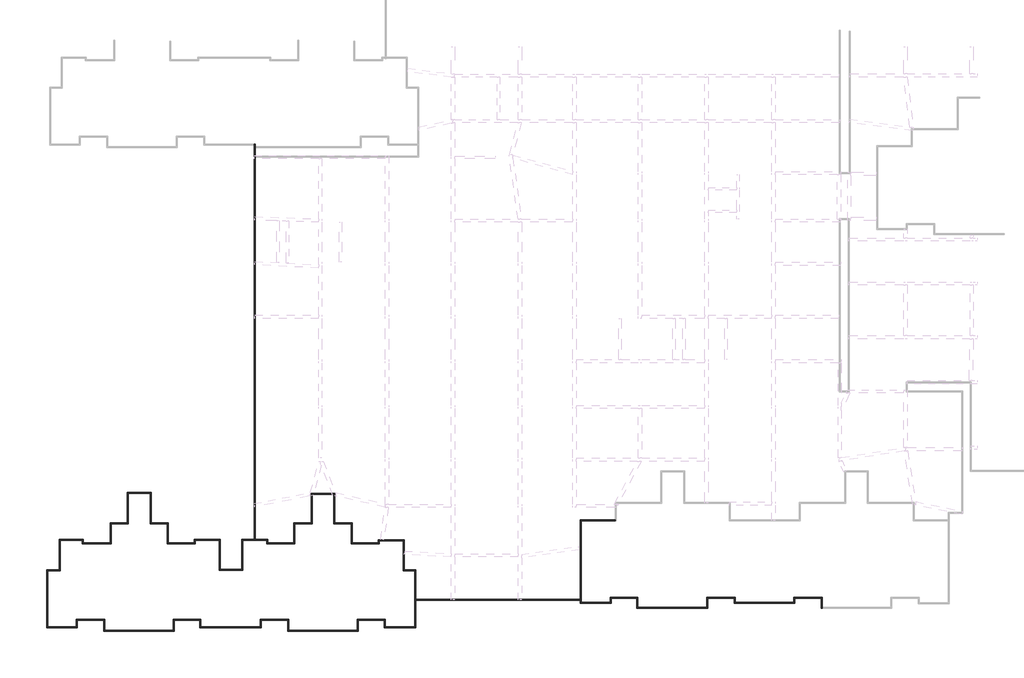
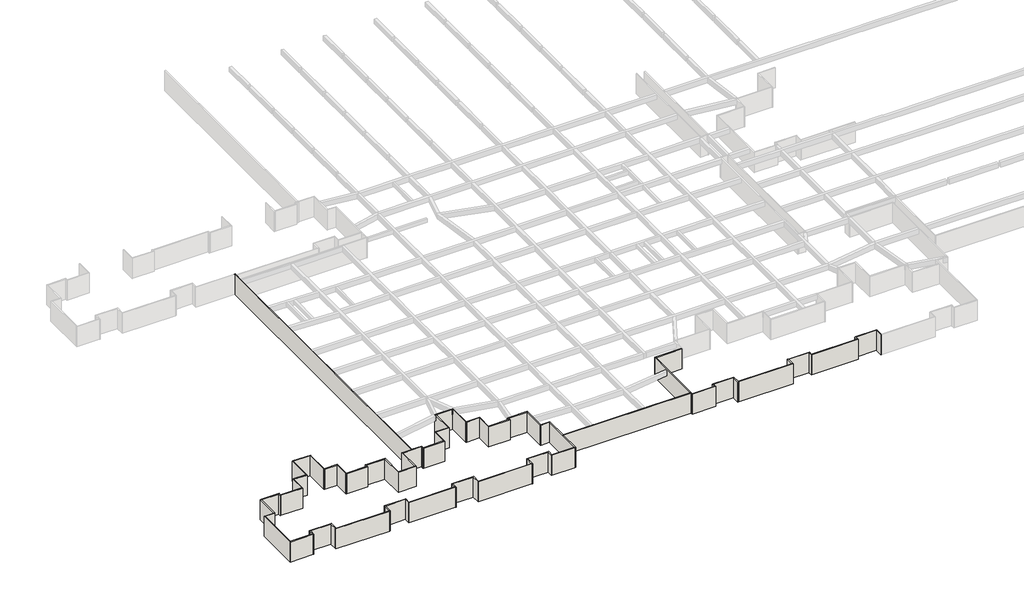
# One storey, part 1 of 16: 68 walls.
"""IFC4 building model written with IfcOpenShell, lengths in millimetres."""

from ifc_helpers import new_model, si_unit, origin, origin_with_axes, place, context, project, spatial, polyline, outline, extrude, faceted_brep, element, save

model = new_model("IFC4")

# Units and contexts
model_context = context("Model", 3, world=origin())
ifc_project = project(units=[si_unit("LENGTHUNIT", "METRE", prefix="MILLI")], contexts=[model_context])

# Site, building, storey
site = spatial("IfcSite", under=ifc_project)
building = spatial("IfcBuilding", under=site)
storey = spatial("IfcBuildingStorey", under=building, Name="户型图", Elevation=0.0)

# Walls
placement = place(None, origin())
element("IfcWall", 1, ObjectType="所有墙体", at=placement, inside=storey, context=model_context, shape_type="Brep", body=[
    faceted_brep([(223706.9772993, -230776.4067791, 0.0), (227415.8823447, -230776.4067791, 0.0), (227415.8823447, -230776.4067791, 3300.0), (223706.9772993, -230776.4067791, 3300.0), (223706.9772993, -230656.4067791, 0.0), (223706.9772993, -230656.4067791, 3300.0), (223826.9772993, -230656.4067791, 3300.0), (227295.8823447, -230656.4067791, 3300.0), (227415.8823447, -230656.4067791, 3300.0), (227415.8823447, -230656.4067791, 0.0), (227295.8823447, -230656.4067791, 0.0), (223826.9772993, -230656.4067791, 0.0)], [[[0, 1, 2, 3]], [[4, 5, 6, 7, 8, 9, 10, 11]], [[1, 0, 4, 11, 10, 9]], [[3, 2, 8, 7, 6, 5]], [[2, 1, 9, 8]], [[0, 3, 5, 4]]]),
])
element("IfcWall", 2, ObjectType="所有墙体", at=placement, inside=storey, context=model_context, shape_type="Brep", body=[
    faceted_brep([(227415.8823447, -230656.4067791, 0.0), (227415.8823447, -230192.9670343, 0.0), (227415.8823447, -230072.9670343, 0.0), (227415.8823447, -230072.9670343, 3300.0), (227415.8823447, -230192.9670343, 3300.0), (227415.8823447, -230656.4067791, 3300.0), (227295.8823447, -230656.4067791, 0.0), (227295.8823447, -230656.4067791, 3300.0), (227295.8823447, -230072.9670343, 3300.0), (227295.8823447, -230072.9670343, 0.0)], [[[0, 1, 2, 3, 4, 5]], [[6, 7, 8, 9]], [[2, 1, 0, 6, 9]], [[5, 4, 3, 8, 7]], [[0, 5, 7, 6]], [[3, 2, 9, 8]]]),
])
element("IfcWall", 3, ObjectType="所有墙体", at=placement, inside=storey, context=model_context, shape_type="Brep", body=[
    faceted_brep([(227415.8823447, -230192.9670343, 0.0), (230497.4582485, -230192.9670343, 0.0), (230617.4582485, -230192.9670343, 0.0), (230617.4582485, -230192.9670343, 3300.0), (230497.4582485, -230192.9670343, 3300.0), (227415.8823447, -230192.9670343, 3300.0), (227415.8823447, -230072.9670343, 0.0), (227415.8823447, -230072.9670343, 3300.0), (230617.4582485, -230072.9670343, 3300.0), (230617.4582485, -230072.9670343, 0.0)], [[[0, 1, 2, 3, 4, 5]], [[6, 7, 8, 9]], [[2, 1, 0, 6, 9]], [[5, 4, 3, 8, 7]], [[0, 5, 7, 6]], [[3, 2, 9, 8]]]),
])
element("IfcWall", 4, ObjectType="所有墙体", at=placement, inside=storey, context=model_context, shape_type="Brep", body=[
    faceted_brep([(230497.4582485, -230192.9670343, 0.0), (230497.4582485, -231395.926057, 0.0), (230497.4582485, -231395.926057, 3300.0), (230497.4582485, -230192.9670343, 3300.0), (230617.4582485, -230192.9670343, 0.0), (230617.4582485, -230192.9670343, 3300.0), (230617.4582485, -231275.926057, 3300.0), (230617.4582485, -231395.926057, 3300.0), (230617.4582485, -231395.926057, 0.0), (230617.4582485, -231275.926057, 0.0)], [[[0, 1, 2, 3]], [[4, 5, 6, 7, 8, 9]], [[1, 0, 4, 9, 8]], [[3, 2, 7, 6, 5]], [[0, 3, 5, 4]], [[2, 1, 8, 7]]]),
])
element("IfcWall", 5, ObjectType="所有墙体", at=placement, inside=storey, context=model_context, shape_type="Brep", body=[
    faceted_brep([(230617.4582485, -231395.926057, 0.0), (239114.4178107, -231395.926057, 0.0), (239114.4178107, -231395.926057, 3300.0), (230617.4582485, -231395.926057, 3300.0), (230617.4582485, -231275.926057, 0.0), (230617.4582485, -231275.926057, 3300.0), (238994.4178107, -231275.926057, 3300.0), (239114.4178107, -231275.926057, 3300.0), (239114.4178107, -231275.926057, 0.0), (238994.4178107, -231275.926057, 0.0)], [[[0, 1, 2, 3]], [[4, 5, 6, 7, 8, 9]], [[1, 0, 4, 9, 8]], [[3, 2, 7, 6, 5]], [[0, 3, 5, 4]], [[2, 1, 8, 7]]]),
])
element("IfcWall", 6, ObjectType="所有墙体", at=placement, inside=storey, context=model_context, shape_type="Brep", body=[
    faceted_brep([(239114.4178107, -231275.926057, 0.0), (239114.4178107, -230192.9670343, 0.0), (239114.4178107, -230072.9670343, 0.0), (239114.4178107, -230072.9670343, 3300.0), (239114.4178107, -230192.9670343, 3300.0), (239114.4178107, -231275.926057, 3300.0), (238994.4178107, -231275.926057, 0.0), (238994.4178107, -231275.926057, 3300.0), (238994.4178107, -230072.9670343, 3300.0), (238994.4178107, -230072.9670343, 0.0)], [[[0, 1, 2, 3, 4, 5]], [[6, 7, 8, 9]], [[2, 1, 0, 6, 9]], [[5, 4, 3, 8, 7]], [[0, 5, 7, 6]], [[3, 2, 9, 8]]]),
])
element("IfcWall", 7, ObjectType="所有墙体", at=placement, inside=storey, context=model_context, shape_type="Brep", body=[
    faceted_brep([(239114.4178107, -230192.9670343, 0.0), (242297.4654708, -230192.9670343, 0.0), (242417.4654708, -230192.9670343, 0.0), (242417.4654708, -230192.9670343, 3300.0), (242297.4654708, -230192.9670343, 3300.0), (239114.4178107, -230192.9670343, 3300.0), (239114.4178107, -230072.9670343, 0.0), (239114.4178107, -230072.9670343, 3300.0), (242417.4654708, -230072.9670343, 3300.0), (242417.4654708, -230072.9670343, 0.0)], [[[0, 1, 2, 3, 4, 5]], [[6, 7, 8, 9]], [[2, 1, 0, 6, 9]], [[5, 4, 3, 8, 7]], [[0, 5, 7, 6]], [[3, 2, 9, 8]]]),
])
element("IfcWall", 8, ObjectType="所有墙体", at=placement, inside=storey, context=model_context, shape_type="Brep", body=[
    faceted_brep([(242297.4654708, -230192.9670343, 0.0), (242297.4654708, -230776.4067791, 0.0), (242297.4654708, -230776.4067791, 3300.0), (242297.4654708, -230192.9670343, 3300.0), (242417.4654708, -230192.9670343, 0.0), (242417.4654708, -230192.9670343, 3300.0), (242417.4654708, -230656.4067791, 3300.0), (242417.4654708, -230776.4067791, 3300.0), (242417.4654708, -230776.4067791, 0.0), (242417.4654708, -230656.4067791, 0.0)], [[[0, 1, 2, 3]], [[4, 5, 6, 7, 8, 9]], [[1, 0, 4, 9, 8]], [[3, 2, 7, 6, 5]], [[0, 3, 5, 4]], [[2, 1, 8, 7]]]),
])
element("IfcWall", 9, ObjectType="所有墙体", at=placement, inside=storey, context=model_context, shape_type="Brep", body=[
    faceted_brep([(242417.4654708, -230776.4067791, 0.0), (249616.6616196, -230776.4067791, 0.0), (249616.6616196, -230776.4067791, 3300.0), (242417.4654708, -230776.4067791, 3300.0), (242417.4654708, -230656.4067791, 0.0), (242417.4654708, -230656.4067791, 3300.0), (249496.6616196, -230656.4067791, 3300.0), (249616.6616196, -230656.4067791, 3300.0), (249616.6616196, -230656.4067791, 0.0), (249496.6616196, -230656.4067791, 0.0)], [[[0, 1, 2, 3]], [[4, 5, 6, 7, 8, 9]], [[1, 0, 4, 9, 8]], [[3, 2, 7, 6, 5]], [[0, 3, 5, 4]], [[2, 1, 8, 7]]]),
])
element("IfcWall", 10, ObjectType="所有墙体", at=placement, inside=storey, context=model_context, shape_type="Brep", body=[
    faceted_brep([(249616.6616196, -230656.4067791, 0.0), (249616.6616196, -230192.9670343, 0.0), (249616.6616196, -230072.9670343, 0.0), (249616.6616196, -230072.9670343, 3300.0), (249616.6616196, -230192.9670343, 3300.0), (249616.6616196, -230656.4067791, 3300.0), (249496.6616196, -230656.4067791, 0.0), (249496.6616196, -230656.4067791, 3300.0), (249496.6616196, -230072.9670343, 3300.0), (249496.6616196, -230072.9670343, 0.0)], [[[0, 1, 2, 3, 4, 5]], [[6, 7, 8, 9]], [[2, 1, 0, 6, 9]], [[5, 4, 3, 8, 7]], [[0, 5, 7, 6]], [[3, 2, 9, 8]]]),
])
element("IfcWall", 11, ObjectType="所有墙体", at=placement, inside=storey, context=model_context, shape_type="Brep", body=[
    faceted_brep([(249616.6616196, -230192.9670343, 0.0), (252797.4720082, -230192.9670343, 0.0), (252917.4720082, -230192.9670343, 0.0), (252917.4720082, -230192.9670343, 3300.0), (252797.4720082, -230192.9670343, 3300.0), (249616.6616196, -230192.9670343, 3300.0), (249616.6616196, -230072.9670343, 0.0), (249616.6616196, -230072.9670343, 3300.0), (252917.4720082, -230072.9670343, 3300.0), (252917.4720082, -230072.9670343, 0.0)], [[[0, 1, 2, 3, 4, 5]], [[6, 7, 8, 9]], [[2, 1, 0, 6, 9]], [[5, 4, 3, 8, 7]], [[0, 5, 7, 6]], [[3, 2, 9, 8]]]),
])
element("IfcWall", 12, ObjectType="所有墙体", at=placement, inside=storey, context=model_context, shape_type="Brep", body=[
    faceted_brep([(252797.4720082, -230192.9670343, 0.0), (252797.4720082, -231395.926057, 0.0), (252797.4720082, -231395.926057, 3300.0), (252797.4720082, -230192.9670343, 3300.0), (252917.4720082, -230192.9670343, 0.0), (252917.4720082, -230192.9670343, 3300.0), (252917.4720082, -231275.926057, 3300.0), (252917.4720082, -231395.926057, 3300.0), (252917.4720082, -231395.926057, 0.0), (252917.4720082, -231275.926057, 0.0)], [[[0, 1, 2, 3]], [[4, 5, 6, 7, 8, 9]], [[1, 0, 4, 9, 8]], [[3, 2, 7, 6, 5]], [[0, 3, 5, 4]], [[2, 1, 8, 7]]]),
])
element("IfcWall", 13, ObjectType="所有墙体", at=placement, inside=storey, context=model_context, shape_type="Brep", body=[
    faceted_brep([(227909.4754658, -220713.7545432, 0.0), (223706.9772993, -220713.7545432, 0.0), (223706.9772993, -220713.7545432, 3300.0), (227909.4754658, -220713.7545432, 3300.0), (227909.4754658, -220833.7545432, 0.0), (227909.4754658, -220833.7545432, 3300.0), (223826.9772993, -220833.7545432, 3300.0), (223706.9772993, -220833.7545432, 3300.0), (223706.9772993, -220833.7545432, 0.0), (223826.9772993, -220833.7545432, 0.0)], [[[0, 1, 2, 3]], [[4, 5, 6, 7, 8, 9]], [[1, 0, 4, 9, 8]], [[3, 2, 7, 6, 5]], [[0, 3, 5, 4]], [[2, 1, 8, 7]]]),
])
element("IfcWall", 14, ObjectType="所有墙体", at=placement, inside=storey, context=model_context, shape_type="Brep", body=[
    faceted_brep([(223706.9772993, -220833.7545432, 0.0), (223706.9772993, -230332.9670343, 0.0), (223706.9772993, -230452.9670343, 0.0), (223706.9772993, -230656.4067791, 0.0), (223706.9772993, -230656.4067791, 3300.0), (223706.9772993, -230452.9670343, 3300.0), (223706.9772993, -230332.9670343, 3300.0), (223706.9772993, -220833.7545432, 3300.0), (223826.9772993, -220833.7545432, 0.0), (223826.9772993, -220833.7545432, 3300.0), (223826.9772993, -230656.4067791, 3300.0), (223826.9772993, -230656.4067791, 0.0)], [[[0, 1, 2, 3, 4, 5, 6, 7]], [[8, 9, 10, 11]], [[3, 2, 1, 0, 8, 11]], [[7, 6, 5, 4, 10, 9]], [[4, 3, 11, 10]], [[0, 7, 9, 8]]]),
])
element("IfcWall", 15, ObjectType="所有墙体", at=placement, inside=storey, context=model_context, shape_type="SweptSolid", body=[
    extrude(outline(polyline([(203826.9772993, -230332.9670343), (223706.9772993, -230332.9670343), (223706.9772993, -230452.9670343), (203826.9772993, -230452.9670343), (203826.9772993, -230332.9670343)])), origin_with_axes(), (0.0, 0.0, 1.0), 3300.0),
])
element("IfcWall", 16, ObjectType="所有墙体", at=placement, inside=storey, context=model_context, shape_type="Brep", body=[
    faceted_brep([(203706.9772993, -226864.0850951, 0.0), (203706.9772993, -233644.4703624, 0.0), (203706.9772993, -233764.4703624, 0.0), (203706.9772993, -233764.4703624, 3300.0), (203706.9772993, -233644.4703624, 3300.0), (203706.9772993, -226864.0850951, 3300.0), (203826.9772993, -226864.0850951, 0.0), (203826.9772993, -226864.0850951, 3300.0), (203826.9772993, -230332.9670343, 3300.0), (203826.9772993, -230452.9670343, 3300.0), (203826.9772993, -233764.4703624, 3300.0), (203826.9772993, -233764.4703624, 0.0), (203826.9772993, -230452.9670343, 0.0), (203826.9772993, -230332.9670343, 0.0)], [[[0, 1, 2, 3, 4, 5]], [[6, 7, 8, 9, 10, 11, 12, 13]], [[2, 1, 0, 6, 13, 12, 11]], [[5, 4, 3, 10, 9, 8, 7]], [[3, 2, 11, 10]], [[0, 5, 7, 6]]]),
])
element("IfcWall", 17, ObjectType="所有墙体", at=placement, inside=storey, context=model_context, shape_type="Brep", body=[
    faceted_brep([(203706.9772993, -233644.4703624, 0.0), (200175.3999887, -233644.4703624, 0.0), (200055.3999887, -233644.4703624, 0.0), (200055.3999887, -233644.4703624, 3300.0), (200175.3999887, -233644.4703624, 3300.0), (203706.9772993, -233644.4703624, 3300.0), (203706.9772993, -233764.4703624, 0.0), (203706.9772993, -233764.4703624, 3300.0), (200055.3999887, -233764.4703624, 3300.0), (200055.3999887, -233764.4703624, 0.0)], [[[0, 1, 2, 3, 4, 5]], [[6, 7, 8, 9]], [[2, 1, 0, 6, 9]], [[5, 4, 3, 8, 7]], [[0, 5, 7, 6]], [[3, 2, 9, 8]]]),
])
element("IfcWall", 18, ObjectType="所有墙体", at=placement, inside=storey, context=model_context, shape_type="Brep", body=[
    faceted_brep([(200175.3999887, -233644.4703624, 0.0), (200175.3999887, -232740.7855886, 0.0), (200175.3999887, -232740.7855886, 3300.0), (200175.3999887, -233644.4703624, 3300.0), (200055.3999887, -233644.4703624, 0.0), (200055.3999887, -233644.4703624, 3300.0), (200055.3999887, -232860.7855886, 3300.0), (200055.3999887, -232740.7855886, 3300.0), (200055.3999887, -232740.7855886, 0.0), (200055.3999887, -232860.7855886, 0.0)], [[[0, 1, 2, 3]], [[4, 5, 6, 7, 8, 9]], [[1, 0, 4, 9, 8]], [[3, 2, 7, 6, 5]], [[0, 3, 5, 4]], [[2, 1, 8, 7]]]),
])
element("IfcWall", 19, ObjectType="所有墙体", at=placement, inside=storey, context=model_context, shape_type="Brep", body=[
    faceted_brep([(200055.3999887, -232740.7855886, 0.0), (196755.597577, -232740.7855886, 0.0), (196755.597577, -232740.7855886, 3300.0), (200055.3999887, -232740.7855886, 3300.0), (200055.3999887, -232860.7855886, 0.0), (200055.3999887, -232860.7855886, 3300.0), (196875.597577, -232860.7855886, 3300.0), (196755.597577, -232860.7855886, 3300.0), (196755.597577, -232860.7855886, 0.0), (196875.597577, -232860.7855886, 0.0)], [[[0, 1, 2, 3]], [[4, 5, 6, 7, 8, 9]], [[1, 0, 4, 9, 8]], [[3, 2, 7, 6, 5]], [[0, 3, 5, 4]], [[2, 1, 8, 7]]]),
])
element("IfcWall", 20, ObjectType="所有墙体", at=placement, inside=storey, context=model_context, shape_type="Brep", body=[
    faceted_brep([(196755.597577, -232860.7855886, 0.0), (196755.597577, -234037.6063178, 0.0), (196755.597577, -234157.6063178, 0.0), (196755.597577, -234157.6063178, 3300.0), (196755.597577, -234037.6063178, 3300.0), (196755.597577, -232860.7855886, 3300.0), (196875.597577, -232860.7855886, 0.0), (196875.597577, -232860.7855886, 3300.0), (196875.597577, -234157.6063178, 3300.0), (196875.597577, -234157.6063178, 0.0)], [[[0, 1, 2, 3, 4, 5]], [[6, 7, 8, 9]], [[2, 1, 0, 6, 9]], [[5, 4, 3, 8, 7]], [[0, 5, 7, 6]], [[3, 2, 9, 8]]]),
])
element("IfcWall", 21, ObjectType="所有墙体", at=placement, inside=storey, context=model_context, shape_type="Brep", body=[
    faceted_brep([(196755.597577, -234037.6063178, 0.0), (188474.9819031, -234037.6063178, 0.0), (188354.9819031, -234037.6063178, 0.0), (188354.9819031, -234037.6063178, 3300.0), (188474.9819031, -234037.6063178, 3300.0), (196755.597577, -234037.6063178, 3300.0), (196755.597577, -234157.6063178, 0.0), (196755.597577, -234157.6063178, 3300.0), (188354.9819031, -234157.6063178, 3300.0), (188354.9819031, -234157.6063178, 0.0)], [[[0, 1, 2, 3, 4, 5]], [[6, 7, 8, 9]], [[2, 1, 0, 6, 9]], [[5, 4, 3, 8, 7]], [[0, 5, 7, 6]], [[3, 2, 9, 8]]]),
])
element("IfcWall", 22, ObjectType="所有墙体", at=placement, inside=storey, context=model_context, shape_type="Brep", body=[
    faceted_brep([(188474.9819031, -234037.6063178, 0.0), (188474.9819031, -232740.7855886, 0.0), (188474.9819031, -232740.7855886, 3300.0), (188474.9819031, -234037.6063178, 3300.0), (188354.9819031, -234037.6063178, 0.0), (188354.9819031, -234037.6063178, 3300.0), (188354.9819031, -232860.7855886, 3300.0), (188354.9819031, -232740.7855886, 3300.0), (188354.9819031, -232740.7855886, 0.0), (188354.9819031, -232860.7855886, 0.0)], [[[0, 1, 2, 3]], [[4, 5, 6, 7, 8, 9]], [[1, 0, 4, 9, 8]], [[3, 2, 7, 6, 5]], [[0, 3, 5, 4]], [[2, 1, 8, 7]]]),
])
element("IfcWall", 23, ObjectType="所有墙体", at=placement, inside=storey, context=model_context, shape_type="Brep", body=[
    faceted_brep([(188354.9819031, -232740.7855886, 0.0), (185055.2276269, -232740.7855886, 0.0), (185055.2276269, -232740.7855886, 3300.0), (188354.9819031, -232740.7855886, 3300.0), (188354.9819031, -232860.7855886, 0.0), (188354.9819031, -232860.7855886, 3300.0), (185175.2276269, -232860.7855886, 3300.0), (185055.2276269, -232860.7855886, 3300.0), (185055.2276269, -232860.7855886, 0.0), (185175.2276269, -232860.7855886, 0.0)], [[[0, 1, 2, 3]], [[4, 5, 6, 7, 8, 9]], [[1, 0, 4, 9, 8]], [[3, 2, 7, 6, 5]], [[0, 3, 5, 4]], [[2, 1, 8, 7]]]),
])
element("IfcWall", 24, ObjectType="所有墙体", at=placement, inside=storey, context=model_context, shape_type="Brep", body=[
    faceted_brep([(185055.2276269, -232860.7855886, 0.0), (185055.2276269, -233644.4703624, 0.0), (185055.2276269, -233764.4703624, 0.0), (185055.2276269, -233764.4703624, 3300.0), (185055.2276269, -233644.4703624, 3300.0), (185055.2276269, -232860.7855886, 3300.0), (185175.2276269, -232860.7855886, 0.0), (185175.2276269, -232860.7855886, 3300.0), (185175.2276269, -233764.4703624, 3300.0), (185175.2276269, -233764.4703624, 0.0)], [[[0, 1, 2, 3, 4, 5]], [[6, 7, 8, 9]], [[2, 1, 0, 6, 9]], [[5, 4, 3, 8, 7]], [[0, 5, 7, 6]], [[3, 2, 9, 8]]]),
])
element("IfcWall", 25, ObjectType="所有墙体", at=placement, inside=storey, context=model_context, shape_type="Brep", body=[
    faceted_brep([(185055.2276269, -233644.4703624, 0.0), (177874.9677687, -233644.4703624, 0.0), (177754.9677687, -233644.4703624, 0.0), (177754.9677687, -233644.4703624, 3300.0), (177874.9677687, -233644.4703624, 3300.0), (185055.2276269, -233644.4703624, 3300.0), (185055.2276269, -233764.4703624, 0.0), (185055.2276269, -233764.4703624, 3300.0), (177754.9677687, -233764.4703624, 3300.0), (177754.9677687, -233764.4703624, 0.0)], [[[0, 1, 2, 3, 4, 5]], [[6, 7, 8, 9]], [[2, 1, 0, 6, 9]], [[5, 4, 3, 8, 7]], [[0, 5, 7, 6]], [[3, 2, 9, 8]]]),
])
element("IfcWall", 26, ObjectType="所有墙体", at=placement, inside=storey, context=model_context, shape_type="Brep", body=[
    faceted_brep([(177874.9677687, -233644.4703624, 0.0), (177874.9677687, -232740.7855886, 0.0), (177874.9677687, -232740.7855886, 3300.0), (177874.9677687, -233644.4703624, 3300.0), (177754.9677687, -233644.4703624, 0.0), (177754.9677687, -233644.4703624, 3300.0), (177754.9677687, -232860.7855886, 3300.0), (177754.9677687, -232740.7855886, 3300.0), (177754.9677687, -232740.7855886, 0.0), (177754.9677687, -232860.7855886, 0.0)], [[[0, 1, 2, 3]], [[4, 5, 6, 7, 8, 9]], [[1, 0, 4, 9, 8]], [[3, 2, 7, 6, 5]], [[0, 3, 5, 4]], [[2, 1, 8, 7]]]),
])
element("IfcWall", 27, ObjectType="所有墙体", at=placement, inside=storey, context=model_context, shape_type="Brep", body=[
    faceted_brep([(177754.9677687, -232740.7855886, 0.0), (174555.583755, -232740.7855886, 0.0), (174555.583755, -232740.7855886, 3300.0), (177754.9677687, -232740.7855886, 3300.0), (177754.9677687, -232860.7855886, 0.0), (177754.9677687, -232860.7855886, 3300.0), (174675.583755, -232860.7855886, 3300.0), (174555.583755, -232860.7855886, 3300.0), (174555.583755, -232860.7855886, 0.0), (174675.583755, -232860.7855886, 0.0)], [[[0, 1, 2, 3]], [[4, 5, 6, 7, 8, 9]], [[1, 0, 4, 9, 8]], [[3, 2, 7, 6, 5]], [[0, 3, 5, 4]], [[2, 1, 8, 7]]]),
])
element("IfcWall", 28, ObjectType="所有墙体", at=placement, inside=storey, context=model_context, shape_type="Brep", body=[
    faceted_brep([(174555.583755, -232860.7855886, 0.0), (174555.583755, -234037.6063178, 0.0), (174555.583755, -234157.6063178, 0.0), (174555.583755, -234157.6063178, 3300.0), (174555.583755, -234037.6063178, 3300.0), (174555.583755, -232860.7855886, 3300.0), (174675.583755, -232860.7855886, 0.0), (174675.583755, -232860.7855886, 3300.0), (174675.583755, -234157.6063178, 3300.0), (174675.583755, -234157.6063178, 0.0)], [[[0, 1, 2, 3, 4, 5]], [[6, 7, 8, 9]], [[2, 1, 0, 6, 9]], [[5, 4, 3, 8, 7]], [[0, 5, 7, 6]], [[3, 2, 9, 8]]]),
])
element("IfcWall", 29, ObjectType="所有墙体", at=placement, inside=storey, context=model_context, shape_type="Brep", body=[
    faceted_brep([(174555.583755, -234037.6063178, 0.0), (166275.583755, -234037.6063178, 0.0), (166155.583755, -234037.6063178, 0.0), (166155.583755, -234037.6063178, 3300.0), (166275.583755, -234037.6063178, 3300.0), (174555.583755, -234037.6063178, 3300.0), (174555.583755, -234157.6063178, 0.0), (174555.583755, -234157.6063178, 3300.0), (166155.583755, -234157.6063178, 3300.0), (166155.583755, -234157.6063178, 0.0)], [[[0, 1, 2, 3, 4, 5]], [[6, 7, 8, 9]], [[2, 1, 0, 6, 9]], [[5, 4, 3, 8, 7]], [[0, 5, 7, 6]], [[3, 2, 9, 8]]]),
])
element("IfcWall", 30, ObjectType="所有墙体", at=placement, inside=storey, context=model_context, shape_type="Brep", body=[
    faceted_brep([(166275.583755, -234037.6063178, 0.0), (166275.583755, -232740.7855886, 0.0), (166275.583755, -232740.7855886, 3300.0), (166275.583755, -234037.6063178, 3300.0), (166155.583755, -234037.6063178, 0.0), (166155.583755, -234037.6063178, 3300.0), (166155.583755, -232860.7855886, 3300.0), (166155.583755, -232740.7855886, 3300.0), (166155.583755, -232740.7855886, 0.0), (166155.583755, -232860.7855886, 0.0)], [[[0, 1, 2, 3]], [[4, 5, 6, 7, 8, 9]], [[1, 0, 4, 9, 8]], [[3, 2, 7, 6, 5]], [[0, 3, 5, 4]], [[2, 1, 8, 7]]]),
])
element("IfcWall", 31, ObjectType="所有墙体", at=placement, inside=storey, context=model_context, shape_type="Brep", body=[
    faceted_brep([(166155.583755, -232740.7855886, 0.0), (162855.771752, -232740.7855886, 0.0), (162855.771752, -232740.7855886, 3300.0), (166155.583755, -232740.7855886, 3300.0), (166155.583755, -232860.7855886, 0.0), (166155.583755, -232860.7855886, 3300.0), (162975.771752, -232860.7855886, 3300.0), (162855.771752, -232860.7855886, 3300.0), (162855.771752, -232860.7855886, 0.0), (162975.771752, -232860.7855886, 0.0)], [[[0, 1, 2, 3]], [[4, 5, 6, 7, 8, 9]], [[1, 0, 4, 9, 8]], [[3, 2, 7, 6, 5]], [[0, 3, 5, 4]], [[2, 1, 8, 7]]]),
])
element("IfcWall", 32, ObjectType="所有墙体", at=placement, inside=storey, context=model_context, shape_type="Brep", body=[
    faceted_brep([(162855.771752, -232860.7855886, 0.0), (162855.771752, -233644.4703624, 0.0), (162855.771752, -233764.4703624, 0.0), (162855.771752, -233764.4703624, 3300.0), (162855.771752, -233644.4703624, 3300.0), (162855.771752, -232860.7855886, 3300.0), (162975.771752, -232860.7855886, 0.0), (162975.771752, -232860.7855886, 3300.0), (162975.771752, -233764.4703624, 3300.0), (162975.771752, -233764.4703624, 0.0)], [[[0, 1, 2, 3, 4, 5]], [[6, 7, 8, 9]], [[2, 1, 0, 6, 9]], [[5, 4, 3, 8, 7]], [[0, 5, 7, 6]], [[3, 2, 9, 8]]]),
])
element("IfcWall", 33, ObjectType="所有墙体", at=placement, inside=storey, context=model_context, shape_type="Brep", body=[
    faceted_brep([(162855.771752, -233644.4703624, 0.0), (159373.4496687, -233644.4703624, 0.0), (159253.4496687, -233644.4703624, 0.0), (159253.4496687, -233644.4703624, 3300.0), (159373.4496687, -233644.4703624, 3300.0), (162855.771752, -233644.4703624, 3300.0), (162855.771752, -233764.4703624, 0.0), (162855.771752, -233764.4703624, 3300.0), (159253.4496687, -233764.4703624, 3300.0), (159253.4496687, -233764.4703624, 0.0)], [[[0, 1, 2, 3, 4, 5]], [[6, 7, 8, 9]], [[2, 1, 0, 6, 9]], [[5, 4, 3, 8, 7]], [[0, 5, 7, 6]], [[3, 2, 9, 8]]]),
])
element("IfcWall", 34, ObjectType="所有墙体", at=placement, inside=storey, context=model_context, shape_type="Brep", body=[
    faceted_brep([(159373.4496687, -233644.4703624, 0.0), (159373.4496687, -226864.4703624, 0.0), (159373.4496687, -226744.4703624, 0.0), (159373.4496687, -226744.4703624, 3300.0), (159373.4496687, -226864.4703624, 3300.0), (159373.4496687, -233644.4703624, 3300.0), (159253.4496687, -233644.4703624, 0.0), (159253.4496687, -233644.4703624, 3300.0), (159253.4496687, -226744.4703624, 3300.0), (159253.4496687, -226744.4703624, 0.0)], [[[0, 1, 2, 3, 4, 5]], [[6, 7, 8, 9]], [[2, 1, 0, 6, 9]], [[5, 4, 3, 8, 7]], [[0, 5, 7, 6]], [[3, 2, 9, 8]]]),
])
element("IfcWall", 35, ObjectType="所有墙体", at=placement, inside=storey, context=model_context, shape_type="Brep", body=[
    faceted_brep([(159373.4496687, -226864.4703624, 0.0), (160883.9958696, -226864.4703624, 0.0), (160883.9958696, -226864.4703624, 3300.0), (159373.4496687, -226864.4703624, 3300.0), (159373.4496687, -226744.4703624, 0.0), (159373.4496687, -226744.4703624, 3300.0), (160763.9958696, -226744.4703624, 3300.0), (160883.9958696, -226744.4703624, 3300.0), (160883.9958696, -226744.4703624, 0.0), (160763.9958696, -226744.4703624, 0.0)], [[[0, 1, 2, 3]], [[4, 5, 6, 7, 8, 9]], [[1, 0, 4, 9, 8]], [[3, 2, 7, 6, 5]], [[0, 3, 5, 4]], [[2, 1, 8, 7]]]),
])
element("IfcWall", 36, ObjectType="所有墙体", at=placement, inside=storey, context=model_context, shape_type="Brep", body=[
    faceted_brep([(160883.9958696, -226744.4703624, 0.0), (160883.9958696, -223216.850594, 0.0), (160883.9958696, -223096.850594, 0.0), (160883.9958696, -223096.850594, 3300.0), (160883.9958696, -223216.850594, 3300.0), (160883.9958696, -226744.4703624, 3300.0), (160763.9958696, -226744.4703624, 0.0), (160763.9958696, -226744.4703624, 3300.0), (160763.9958696, -223096.850594, 3300.0), (160763.9958696, -223096.850594, 0.0)], [[[0, 1, 2, 3, 4, 5]], [[6, 7, 8, 9]], [[2, 1, 0, 6, 9]], [[5, 4, 3, 8, 7]], [[0, 5, 7, 6]], [[3, 2, 9, 8]]]),
])
element("IfcWall", 37, ObjectType="所有墙体", at=placement, inside=storey, context=model_context, shape_type="Brep", body=[
    faceted_brep([(160883.9958696, -223216.850594, 0.0), (163563.9958696, -223216.850594, 0.0), (163683.9958696, -223216.850594, 0.0), (163683.9958696, -223216.850594, 3300.0), (163563.9958696, -223216.850594, 3300.0), (160883.9958696, -223216.850594, 3300.0), (160883.9958696, -223096.850594, 0.0), (160883.9958696, -223096.850594, 3300.0), (163683.9958696, -223096.850594, 3300.0), (163683.9958696, -223096.850594, 0.0)], [[[0, 1, 2, 3, 4, 5]], [[6, 7, 8, 9]], [[2, 1, 0, 6, 9]], [[5, 4, 3, 8, 7]], [[0, 5, 7, 6]], [[3, 2, 9, 8]]]),
])
element("IfcWall", 38, ObjectType="所有墙体", at=placement, inside=storey, context=model_context, shape_type="Brep", body=[
    faceted_brep([(163563.9958696, -223216.850594, 0.0), (163563.9958696, -223622.1234451, 0.0), (163563.9958696, -223622.1234451, 3300.0), (163563.9958696, -223216.850594, 3300.0), (163683.9958696, -223216.850594, 0.0), (163683.9958696, -223216.850594, 3300.0), (163683.9958696, -223502.1234451, 3300.0), (163683.9958696, -223622.1234451, 3300.0), (163683.9958696, -223622.1234451, 0.0), (163683.9958696, -223502.1234451, 0.0)], [[[0, 1, 2, 3]], [[4, 5, 6, 7, 8, 9]], [[1, 0, 4, 9, 8]], [[3, 2, 7, 6, 5]], [[0, 3, 5, 4]], [[2, 1, 8, 7]]]),
])
element("IfcWall", 39, ObjectType="所有墙体", at=placement, inside=storey, context=model_context, shape_type="Brep", body=[
    faceted_brep([(163683.9958696, -223622.1234451, 0.0), (167083.9958696, -223622.1234451, 0.0), (167083.9958696, -223622.1234451, 3300.0), (163683.9958696, -223622.1234451, 3300.0), (163683.9958696, -223502.1234451, 0.0), (163683.9958696, -223502.1234451, 3300.0), (166963.9958696, -223502.1234451, 3300.0), (167083.9958696, -223502.1234451, 3300.0), (167083.9958696, -223502.1234451, 0.0), (166963.9958696, -223502.1234451, 0.0)], [[[0, 1, 2, 3]], [[4, 5, 6, 7, 8, 9]], [[1, 0, 4, 9, 8]], [[3, 2, 7, 6, 5]], [[0, 3, 5, 4]], [[2, 1, 8, 7]]]),
])
element("IfcWall", 40, ObjectType="所有墙体", at=placement, inside=storey, context=model_context, shape_type="Brep", body=[
    faceted_brep([(167083.9958696, -223502.1234451, 0.0), (167083.9958696, -221223.7957944, 0.0), (167083.9958696, -221103.7957944, 0.0), (167083.9958696, -221103.7957944, 3300.0), (167083.9958696, -221223.7957944, 3300.0), (167083.9958696, -223502.1234451, 3300.0), (166963.9958696, -223502.1234451, 0.0), (166963.9958696, -223502.1234451, 3300.0), (166963.9958696, -221103.7957944, 3300.0), (166963.9958696, -221103.7957944, 0.0)], [[[0, 1, 2, 3, 4, 5]], [[6, 7, 8, 9]], [[2, 1, 0, 6, 9]], [[5, 4, 3, 8, 7]], [[0, 5, 7, 6]], [[3, 2, 9, 8]]]),
])
element("IfcWall", 41, ObjectType="所有墙体", at=placement, inside=storey, context=model_context, shape_type="Brep", body=[
    faceted_brep([(167083.9958696, -221223.7957944, 0.0), (169140.5185226, -221223.7957944, 0.0), (169140.5185226, -221223.7957944, 3300.0), (167083.9958696, -221223.7957944, 3300.0), (167083.9958696, -221103.7957944, 0.0), (167083.9958696, -221103.7957944, 3300.0), (169020.5185226, -221103.7957944, 3300.0), (169140.5185226, -221103.7957944, 3300.0), (169140.5185226, -221103.7957944, 0.0), (169020.5185226, -221103.7957944, 0.0)], [[[0, 1, 2, 3]], [[4, 5, 6, 7, 8, 9]], [[1, 0, 4, 9, 8]], [[3, 2, 7, 6, 5]], [[0, 3, 5, 4]], [[2, 1, 8, 7]]]),
])
element("IfcWall", 42, ObjectType="所有墙体", at=placement, inside=storey, context=model_context, shape_type="Brep", body=[
    faceted_brep([(169140.5185226, -221103.7957944, 0.0), (169140.5185226, -217528.1551832, 0.0), (169140.5185226, -217408.1551832, 0.0), (169140.5185226, -217408.1551832, 3300.0), (169140.5185226, -217528.1551832, 3300.0), (169140.5185226, -221103.7957944, 3300.0), (169020.5185226, -221103.7957944, 0.0), (169020.5185226, -221103.7957944, 3300.0), (169020.5185226, -217408.1551832, 3300.0), (169020.5185226, -217408.1551832, 0.0)], [[[0, 1, 2, 3, 4, 5]], [[6, 7, 8, 9]], [[2, 1, 0, 6, 9]], [[5, 4, 3, 8, 7]], [[0, 5, 7, 6]], [[3, 2, 9, 8]]]),
])
element("IfcWall", 43, ObjectType="所有墙体", at=placement, inside=storey, context=model_context, shape_type="Brep", body=[
    faceted_brep([(169140.5185226, -217528.1551832, 0.0), (171768.3939286, -217528.1551832, 0.0), (171888.3939286, -217528.1551832, 0.0), (171888.3939286, -217528.1551832, 3300.0), (171768.3939286, -217528.1551832, 3300.0), (169140.5185226, -217528.1551832, 3300.0), (169140.5185226, -217408.1551832, 0.0), (169140.5185226, -217408.1551832, 3300.0), (171888.3939286, -217408.1551832, 3300.0), (171888.3939286, -217408.1551832, 0.0)], [[[0, 1, 2, 3, 4, 5]], [[6, 7, 8, 9]], [[2, 1, 0, 6, 9]], [[5, 4, 3, 8, 7]], [[0, 5, 7, 6]], [[3, 2, 9, 8]]]),
])
element("IfcWall", 44, ObjectType="所有墙体", at=placement, inside=storey, context=model_context, shape_type="Brep", body=[
    faceted_brep([(171768.3939286, -217528.1551832, 0.0), (171768.3939286, -221223.7957944, 0.0), (171768.3939286, -221223.7957944, 3300.0), (171768.3939286, -217528.1551832, 3300.0), (171888.3939286, -217528.1551832, 0.0), (171888.3939286, -217528.1551832, 3300.0), (171888.3939286, -221103.7957944, 3300.0), (171888.3939286, -221223.7957944, 3300.0), (171888.3939286, -221223.7957944, 0.0), (171888.3939286, -221103.7957944, 0.0)], [[[0, 1, 2, 3]], [[4, 5, 6, 7, 8, 9]], [[1, 0, 4, 9, 8]], [[3, 2, 7, 6, 5]], [[0, 3, 5, 4]], [[2, 1, 8, 7]]]),
])
element("IfcWall", 45, ObjectType="所有墙体", at=placement, inside=storey, context=model_context, shape_type="Brep", body=[
    faceted_brep([(171888.3939286, -221223.7957944, 0.0), (173817.5367432, -221223.7957944, 0.0), (173937.5367432, -221223.7957944, 0.0), (173937.5367432, -221223.7957944, 3300.0), (173817.5367432, -221223.7957944, 3300.0), (171888.3939286, -221223.7957944, 3300.0), (171888.3939286, -221103.7957944, 0.0), (171888.3939286, -221103.7957944, 3300.0), (173937.5367432, -221103.7957944, 3300.0), (173937.5367432, -221103.7957944, 0.0)], [[[0, 1, 2, 3, 4, 5]], [[6, 7, 8, 9]], [[2, 1, 0, 6, 9]], [[5, 4, 3, 8, 7]], [[0, 5, 7, 6]], [[3, 2, 9, 8]]]),
])
element("IfcWall", 46, ObjectType="所有墙体", at=placement, inside=storey, context=model_context, shape_type="Brep", body=[
    faceted_brep([(173817.5367432, -221223.7957944, 0.0), (173817.5367432, -223622.1234451, 0.0), (173817.5367432, -223622.1234451, 3300.0), (173817.5367432, -221223.7957944, 3300.0), (173937.5367432, -221223.7957944, 0.0), (173937.5367432, -221223.7957944, 3300.0), (173937.5367432, -223502.1234451, 3300.0), (173937.5367432, -223622.1234451, 3300.0), (173937.5367432, -223622.1234451, 0.0), (173937.5367432, -223502.1234451, 0.0)], [[[0, 1, 2, 3]], [[4, 5, 6, 7, 8, 9]], [[1, 0, 4, 9, 8]], [[3, 2, 7, 6, 5]], [[0, 3, 5, 4]], [[2, 1, 8, 7]]]),
])
element("IfcWall", 47, ObjectType="所有墙体", at=placement, inside=storey, context=model_context, shape_type="Brep", body=[
    faceted_brep([(173937.5367432, -223622.1234451, 0.0), (177235.7830045, -223622.1234451, 0.0), (177235.7830045, -223622.1234451, 3300.0), (173937.5367432, -223622.1234451, 3300.0), (173937.5367432, -223502.1234451, 0.0), (173937.5367432, -223502.1234451, 3300.0), (177115.7830045, -223502.1234451, 3300.0), (177235.7830045, -223502.1234451, 3300.0), (177235.7830045, -223502.1234451, 0.0), (177115.7830045, -223502.1234451, 0.0)], [[[0, 1, 2, 3]], [[4, 5, 6, 7, 8, 9]], [[1, 0, 4, 9, 8]], [[3, 2, 7, 6, 5]], [[0, 3, 5, 4]], [[2, 1, 8, 7]]]),
])
element("IfcWall", 48, ObjectType="所有墙体", at=placement, inside=storey, context=model_context, shape_type="Brep", body=[
    faceted_brep([(177235.7830045, -223502.1234451, 0.0), (177235.7830045, -223216.850594, 0.0), (177235.7830045, -223096.850594, 0.0), (177235.7830045, -223096.850594, 3300.0), (177235.7830045, -223216.850594, 3300.0), (177235.7830045, -223502.1234451, 3300.0), (177115.7830045, -223502.1234451, 0.0), (177115.7830045, -223502.1234451, 3300.0), (177115.7830045, -223096.850594, 3300.0), (177115.7830045, -223096.850594, 0.0)], [[[0, 1, 2, 3, 4, 5]], [[6, 7, 8, 9]], [[2, 1, 0, 6, 9]], [[5, 4, 3, 8, 7]], [[0, 5, 7, 6]], [[3, 2, 9, 8]]]),
])
element("IfcWall", 49, ObjectType="所有墙体", at=placement, inside=storey, context=model_context, shape_type="Brep", body=[
    faceted_brep([(177235.7830045, -223216.850594, 0.0), (180116.2371142, -223216.850594, 0.0), (180236.2371142, -223216.850594, 0.0), (180236.2371142, -223216.850594, 3300.0), (180116.2371142, -223216.850594, 3300.0), (177235.7830045, -223216.850594, 3300.0), (177235.7830045, -223096.850594, 0.0), (177235.7830045, -223096.850594, 3300.0), (180236.2371142, -223096.850594, 3300.0), (180236.2371142, -223096.850594, 0.0)], [[[0, 1, 2, 3, 4, 5]], [[6, 7, 8, 9]], [[2, 1, 0, 6, 9]], [[5, 4, 3, 8, 7]], [[0, 5, 7, 6]], [[3, 2, 9, 8]]]),
])
element("IfcWall", 50, ObjectType="所有墙体", at=placement, inside=storey, context=model_context, shape_type="Brep", body=[
    faceted_brep([(180116.2371142, -223216.850594, 0.0), (180116.2371142, -226838.699103, 0.0), (180116.2371142, -226838.699103, 3300.0), (180116.2371142, -223216.850594, 3300.0), (180236.2371142, -223216.850594, 0.0), (180236.2371142, -223216.850594, 3300.0), (180236.2371142, -226718.699103, 3300.0), (180236.2371142, -226838.699103, 3300.0), (180236.2371142, -226838.699103, 0.0), (180236.2371142, -226718.699103, 0.0)], [[[0, 1, 2, 3]], [[4, 5, 6, 7, 8, 9]], [[1, 0, 4, 9, 8]], [[3, 2, 7, 6, 5]], [[0, 3, 5, 4]], [[2, 1, 8, 7]]]),
])
element("IfcWall", 51, ObjectType="所有墙体", at=placement, inside=storey, context=model_context, shape_type="Brep", body=[
    faceted_brep([(180236.2371142, -226838.699103, 0.0), (182932.1971931, -226838.699103, 0.0), (182932.1971931, -226838.699103, 3300.0), (180236.2371142, -226838.699103, 3300.0), (180236.2371142, -226718.699103, 0.0), (180236.2371142, -226718.699103, 3300.0), (182812.1971931, -226718.699103, 3300.0), (182932.1971931, -226718.699103, 3300.0), (182932.1971931, -226718.699103, 0.0), (182812.1971931, -226718.699103, 0.0)], [[[0, 1, 2, 3]], [[4, 5, 6, 7, 8, 9]], [[1, 0, 4, 9, 8]], [[3, 2, 7, 6, 5]], [[0, 3, 5, 4]], [[2, 1, 8, 7]]]),
])
element("IfcWall", 52, ObjectType="所有墙体", at=placement, inside=storey, context=model_context, shape_type="Brep", body=[
    faceted_brep([(182932.1971931, -226718.699103, 0.0), (182932.1971931, -223216.850594, 0.0), (182932.1971931, -223096.850594, 0.0), (182932.1971931, -223096.850594, 3300.0), (182932.1971931, -223216.850594, 3300.0), (182932.1971931, -226718.699103, 3300.0), (182812.1971931, -226718.699103, 0.0), (182812.1971931, -226718.699103, 3300.0), (182812.1971931, -223096.850594, 3300.0), (182812.1971931, -223096.850594, 0.0)], [[[0, 1, 2, 3, 4, 5]], [[6, 7, 8, 9]], [[2, 1, 0, 6, 9]], [[5, 4, 3, 8, 7]], [[0, 5, 7, 6]], [[3, 2, 9, 8]]]),
])
element("IfcWall", 53, ObjectType="所有墙体", at=placement, inside=storey, context=model_context, shape_type="Brep", body=[
    faceted_brep([(182932.1971931, -223216.850594, 0.0), (185816.2406631, -223216.850594, 0.0), (185936.2406631, -223216.850594, 0.0), (185936.2406631, -223216.850594, 3300.0), (185816.2406631, -223216.850594, 3300.0), (182932.1971931, -223216.850594, 3300.0), (182932.1971931, -223096.850594, 0.0), (182932.1971931, -223096.850594, 3300.0), (184314.2189281, -223096.850594, 3300.0), (184434.2189281, -223096.850594, 3300.0), (185936.2406631, -223096.850594, 3300.0), (185936.2406631, -223096.850594, 0.0), (184434.2189281, -223096.850594, 0.0), (184314.2189281, -223096.850594, 0.0)], [[[0, 1, 2, 3, 4, 5]], [[6, 7, 8, 9, 10, 11, 12, 13]], [[2, 1, 0, 6, 13, 12, 11]], [[5, 4, 3, 10, 9, 8, 7]], [[0, 5, 7, 6]], [[3, 2, 11, 10]]]),
])
element("IfcWall", 54, ObjectType="所有墙体", at=placement, inside=storey, context=model_context, shape_type="Brep", body=[
    faceted_brep([(185816.2406631, -223216.850594, 0.0), (185816.2406631, -223622.1234451, 0.0), (185816.2406631, -223622.1234451, 3300.0), (185816.2406631, -223216.850594, 3300.0), (185936.2406631, -223216.850594, 0.0), (185936.2406631, -223216.850594, 3300.0), (185936.2406631, -223502.1234451, 3300.0), (185936.2406631, -223622.1234451, 3300.0), (185936.2406631, -223622.1234451, 0.0), (185936.2406631, -223502.1234451, 0.0)], [[[0, 1, 2, 3]], [[4, 5, 6, 7, 8, 9]], [[1, 0, 4, 9, 8]], [[3, 2, 7, 6, 5]], [[0, 3, 5, 4]], [[2, 1, 8, 7]]]),
])
element("IfcWall", 55, ObjectType="所有墙体", at=placement, inside=storey, context=model_context, shape_type="Brep", body=[
    faceted_brep([(185936.2406631, -223622.1234451, 0.0), (189235.7607746, -223622.1234451, 0.0), (189235.7607746, -223622.1234451, 3300.0), (185936.2406631, -223622.1234451, 3300.0), (185936.2406631, -223502.1234451, 0.0), (185936.2406631, -223502.1234451, 3300.0), (189115.7607746, -223502.1234451, 3300.0), (189235.7607746, -223502.1234451, 3300.0), (189235.7607746, -223502.1234451, 0.0), (189115.7607746, -223502.1234451, 0.0)], [[[0, 1, 2, 3]], [[4, 5, 6, 7, 8, 9]], [[1, 0, 4, 9, 8]], [[3, 2, 7, 6, 5]], [[0, 3, 5, 4]], [[2, 1, 8, 7]]]),
])
element("IfcWall", 56, ObjectType="所有墙体", at=placement, inside=storey, context=model_context, shape_type="Brep", body=[
    faceted_brep([(189235.7607746, -223502.1234451, 0.0), (189235.7607746, -221223.7957944, 0.0), (189235.7607746, -221103.7957944, 0.0), (189235.7607746, -221103.7957944, 3300.0), (189235.7607746, -221223.7957944, 3300.0), (189235.7607746, -223502.1234451, 3300.0), (189115.7607746, -223502.1234451, 0.0), (189115.7607746, -223502.1234451, 3300.0), (189115.7607746, -221103.7957944, 3300.0), (189115.7607746, -221103.7957944, 0.0)], [[[0, 1, 2, 3, 4, 5]], [[6, 7, 8, 9]], [[2, 1, 0, 6, 9]], [[5, 4, 3, 8, 7]], [[0, 5, 7, 6]], [[3, 2, 9, 8]]]),
])
element("IfcWall", 57, ObjectType="所有墙体", at=placement, inside=storey, context=model_context, shape_type="Brep", body=[
    faceted_brep([(189235.7607746, -221223.7957944, 0.0), (191338.4680648, -221223.7957944, 0.0), (191338.4680648, -221223.7957944, 3300.0), (189235.7607746, -221223.7957944, 3300.0), (189235.7607746, -221103.7957944, 0.0), (189235.7607746, -221103.7957944, 3300.0), (191218.4680648, -221103.7957944, 3300.0), (191338.4680648, -221103.7957944, 3300.0), (191338.4680648, -221103.7957944, 0.0), (191218.4680648, -221103.7957944, 0.0)], [[[0, 1, 2, 3]], [[4, 5, 6, 7, 8, 9]], [[1, 0, 4, 9, 8]], [[3, 2, 7, 6, 5]], [[0, 3, 5, 4]], [[2, 1, 8, 7]]]),
])
element("IfcWall", 58, ObjectType="所有墙体", at=placement, inside=storey, context=model_context, shape_type="Brep", body=[
    faceted_brep([(191338.4680648, -221103.7957944, 0.0), (191338.4680648, -217650.8034485, 0.0), (191338.4680648, -217530.8034485, 0.0), (191338.4680648, -217530.8034485, 3300.0), (191338.4680648, -217650.8034485, 3300.0), (191338.4680648, -221103.7957944, 3300.0), (191218.4680648, -221103.7957944, 0.0), (191218.4680648, -221103.7957944, 3300.0), (191218.4680648, -217530.8034485, 3300.0), (191218.4680648, -217530.8034485, 0.0)], [[[0, 1, 2, 3, 4, 5]], [[6, 7, 8, 9]], [[2, 1, 0, 6, 9]], [[5, 4, 3, 8, 7]], [[0, 5, 7, 6]], [[3, 2, 9, 8]]]),
])
element("IfcWall", 59, ObjectType="所有墙体", at=placement, inside=storey, context=model_context, shape_type="Brep", body=[
    faceted_brep([(191338.4680648, -217650.8034485, 0.0), (193922.0585089, -217650.8034485, 0.0), (194042.0585089, -217650.8034485, 0.0), (194042.0585089, -217650.8034485, 3300.0), (193922.0585089, -217650.8034485, 3300.0), (191338.4680648, -217650.8034485, 3300.0), (191338.4680648, -217530.8034485, 0.0), (191338.4680648, -217530.8034485, 3300.0), (194042.0585089, -217530.8034485, 3300.0), (194042.0585089, -217530.8034485, 0.0)], [[[0, 1, 2, 3, 4, 5]], [[6, 7, 8, 9]], [[2, 1, 0, 6, 9]], [[5, 4, 3, 8, 7]], [[0, 5, 7, 6]], [[3, 2, 9, 8]]]),
])
element("IfcWall", 60, ObjectType="所有墙体", at=placement, inside=storey, context=model_context, shape_type="Brep", body=[
    faceted_brep([(193922.0585089, -217650.8034485, 0.0), (193922.0585089, -221223.7957944, 0.0), (193922.0585089, -221223.7957944, 3300.0), (193922.0585089, -217650.8034485, 3300.0), (194042.0585089, -217650.8034485, 0.0), (194042.0585089, -217650.8034485, 3300.0), (194042.0585089, -221103.7957944, 3300.0), (194042.0585089, -221223.7957944, 3300.0), (194042.0585089, -221223.7957944, 0.0), (194042.0585089, -221103.7957944, 0.0)], [[[0, 1, 2, 3]], [[4, 5, 6, 7, 8, 9]], [[1, 0, 4, 9, 8]], [[3, 2, 7, 6, 5]], [[0, 3, 5, 4]], [[2, 1, 8, 7]]]),
])
element("IfcWall", 61, ObjectType="所有墙体", at=placement, inside=storey, context=model_context, shape_type="Brep", body=[
    faceted_brep([(194042.0585089, -221223.7957944, 0.0), (196018.4710534, -221223.7957944, 0.0), (196138.4710534, -221223.7957944, 0.0), (196138.4710534, -221223.7957944, 3300.0), (196018.4710534, -221223.7957944, 3300.0), (194042.0585089, -221223.7957944, 3300.0), (194042.0585089, -221103.7957944, 0.0), (194042.0585089, -221103.7957944, 3300.0), (196138.4710534, -221103.7957944, 3300.0), (196138.4710534, -221103.7957944, 0.0)], [[[0, 1, 2, 3, 4, 5]], [[6, 7, 8, 9]], [[2, 1, 0, 6, 9]], [[5, 4, 3, 8, 7]], [[0, 5, 7, 6]], [[3, 2, 9, 8]]]),
])
element("IfcWall", 62, ObjectType="所有墙体", at=placement, inside=storey, context=model_context, shape_type="Brep", body=[
    faceted_brep([(196018.4710534, -221223.7957944, 0.0), (196018.4710534, -223622.1234451, 0.0), (196018.4710534, -223622.1234451, 3300.0), (196018.4710534, -221223.7957944, 3300.0), (196138.4710534, -221223.7957944, 0.0), (196138.4710534, -221223.7957944, 3300.0), (196138.4710534, -223502.1234451, 3300.0), (196138.4710534, -223622.1234451, 3300.0), (196138.4710534, -223622.1234451, 0.0), (196138.4710534, -223502.1234451, 0.0)], [[[0, 1, 2, 3]], [[4, 5, 6, 7, 8, 9]], [[1, 0, 4, 9, 8]], [[3, 2, 7, 6, 5]], [[0, 3, 5, 4]], [[2, 1, 8, 7]]]),
])
element("IfcWall", 63, ObjectType="所有墙体", at=placement, inside=storey, context=model_context, shape_type="Brep", body=[
    faceted_brep([(196138.4710534, -223622.1234451, 0.0), (199435.7968264, -223622.1234451, 0.0), (199435.7968264, -223622.1234451, 3300.0), (196138.4710534, -223622.1234451, 3300.0), (196138.4710534, -223502.1234451, 0.0), (196138.4710534, -223502.1234451, 3300.0), (199315.7968264, -223502.1234451, 3300.0), (199435.7968264, -223502.1234451, 3300.0), (199435.7968264, -223502.1234451, 0.0), (199315.7968264, -223502.1234451, 0.0)], [[[0, 1, 2, 3]], [[4, 5, 6, 7, 8, 9]], [[1, 0, 4, 9, 8]], [[3, 2, 7, 6, 5]], [[0, 3, 5, 4]], [[2, 1, 8, 7]]]),
])
element("IfcWall", 64, ObjectType="所有墙体", at=placement, inside=storey, context=model_context, shape_type="Brep", body=[
    faceted_brep([(199435.7968264, -223502.1234451, 0.0), (199435.7968264, -223259.2388283, 0.0), (199435.7968264, -223139.2388283, 0.0), (199435.7968264, -223139.2388283, 3300.0), (199435.7968264, -223259.2388283, 3300.0), (199435.7968264, -223502.1234451, 3300.0), (199315.7968264, -223502.1234451, 0.0), (199315.7968264, -223502.1234451, 3300.0), (199315.7968264, -223139.2388283, 3300.0), (199315.7968264, -223139.2388283, 0.0)], [[[0, 1, 2, 3, 4, 5]], [[6, 7, 8, 9]], [[2, 1, 0, 6, 9]], [[5, 4, 3, 8, 7]], [[0, 5, 7, 6]], [[3, 2, 9, 8]]]),
])
element("IfcWall", 65, ObjectType="所有墙体", at=placement, inside=storey, context=model_context, shape_type="Brep", body=[
    faceted_brep([(199435.7968264, -223259.2388283, 0.0), (202315.7968264, -223259.2388283, 0.0), (202435.7968264, -223259.2388283, 0.0), (202435.7968264, -223259.2388283, 3300.0), (202315.7968264, -223259.2388283, 3300.0), (199435.7968264, -223259.2388283, 3300.0), (199435.7968264, -223139.2388283, 0.0), (199435.7968264, -223139.2388283, 3300.0), (202435.7968264, -223139.2388283, 3300.0), (202435.7968264, -223139.2388283, 0.0)], [[[0, 1, 2, 3, 4, 5]], [[6, 7, 8, 9]], [[2, 1, 0, 6, 9]], [[5, 4, 3, 8, 7]], [[0, 5, 7, 6]], [[3, 2, 9, 8]]]),
])
element("IfcWall", 66, ObjectType="所有墙体", at=placement, inside=storey, context=model_context, shape_type="Brep", body=[
    faceted_brep([(202315.7968264, -223259.2388283, 0.0), (202315.7968264, -226864.0850951, 0.0), (202315.7968264, -226864.0850951, 3300.0), (202315.7968264, -223259.2388283, 3300.0), (202435.7968264, -223259.2388283, 0.0), (202435.7968264, -223259.2388283, 3300.0), (202435.7968264, -226744.0850951, 3300.0), (202435.7968264, -226864.0850951, 3300.0), (202435.7968264, -226864.0850951, 0.0), (202435.7968264, -226744.0850951, 0.0)], [[[0, 1, 2, 3]], [[4, 5, 6, 7, 8, 9]], [[1, 0, 4, 9, 8]], [[3, 2, 7, 6, 5]], [[0, 3, 5, 4]], [[2, 1, 8, 7]]]),
])
element("IfcWall", 67, ObjectType="所有墙体", at=placement, inside=storey, context=model_context, shape_type="Brep", body=[
    faceted_brep([(202435.7968264, -226864.0850951, 0.0), (203706.9772993, -226864.0850951, 0.0), (203826.9772993, -226864.0850951, 0.0), (203826.9772993, -226864.0850951, 3300.0), (203706.9772993, -226864.0850951, 3300.0), (202435.7968264, -226864.0850951, 3300.0), (202435.7968264, -226744.0850951, 0.0), (202435.7968264, -226744.0850951, 3300.0), (203826.9772993, -226744.0850951, 3300.0), (203826.9772993, -226744.0850951, 0.0)], [[[0, 1, 2, 3, 4, 5]], [[6, 7, 8, 9]], [[2, 1, 0, 6, 9]], [[5, 4, 3, 8, 7]], [[0, 5, 7, 6]], [[3, 2, 9, 8]]]),
])
element("IfcWall", 68, ObjectType="所有墙体", at=placement, inside=storey, context=model_context, shape_type="Brep", body=[
    faceted_brep([(184434.2189281, -223096.850594, 0.0), (184434.2189281, -176865.1471774, 0.0), (184434.2189281, -176745.1471774, 0.0), (184434.2189281, -175750.7737405, 0.0), (184434.2189281, -175630.7737405, 0.0), (184434.2189281, -175296.850594, 0.0), (184434.2189281, -175296.850594, 3300.0), (184434.2189281, -175630.7737405, 3300.0), (184434.2189281, -175750.7737405, 3300.0), (184434.2189281, -176745.1471774, 3300.0), (184434.2189281, -176865.1471774, 3300.0), (184434.2189281, -223096.850594, 3300.0), (184314.2189281, -223096.850594, 0.0), (184314.2189281, -223096.850594, 3300.0), (184314.2189281, -175416.850594, 3300.0), (184314.2189281, -175296.850594, 3300.0), (184314.2189281, -175296.850594, 0.0), (184314.2189281, -175416.850594, 0.0)], [[[0, 1, 2, 3, 4, 5, 6, 7, 8, 9, 10, 11]], [[12, 13, 14, 15, 16, 17]], [[5, 4, 3, 2, 1, 0, 12, 17, 16]], [[11, 10, 9, 8, 7, 6, 15, 14, 13]], [[0, 11, 13, 12]], [[6, 5, 16, 15]]]),
])

save(model, "model.ifc")

# Revit data of these elements
# Project information
#   项目发布日期 = "出图日期"
#   项目状态 = "项目状态"
#   客户姓名 = "所有者"
#   项目地址 = "## 街道\n省市自治区邮政编码"
#   项目名称 = "项目名称"
#   项目编号 = "项目编号"
# Type "所有墙体"
#   Layers, outside or top first: 120 mm "默认" (function 1)
# Elements 1, 2, 3, 4, 5, 6, 7, 8, 9, 10, 11, 12, 13, 14, 15, 16, 17, 18, 19, 20, 21, 22, 23, 24, 25, 26, 27, 28, 29, 30, 31, 32, 33, 34, 35, 36, 37, 38, 39, 40, 41, 42, 43, 44, 45, 46, 47, 48, 49, 50, 51, 52, 53, 54, 55, 56, 57, 58, 59, 60, 61, 62, 63, 64, 65, 66, 67, 68 (IfcWall, "所有墙体")
#   Top Offset = 0 mm
#   Base Offset = 0 mm
#   wall height = 3300 mm
#   Phase Created = 新构造
#   Base Constraint = 户型图
#   Top Constraint = 层高
#   Materials on its faces: "默认"
# Materials
#   "默认": class "其他", colour RGB 192 192 192, transparency 0, Cost = 0
# Area at (183573.558, -170449.512) mm, upper offset 0 mm, lower offset 0 mm
#   Number = "170"
#   Name = "main_building"
# Area, not placed, upper offset 0 mm, lower offset 0 mm
#   Number = "80"
#   Name = "main_building"
# Area, not placed, upper offset 0 mm, lower offset 0 mm
#   Number = "118"
#   Name = "main_building"
# Area, not placed, upper offset 0 mm, lower offset 0 mm
#   Number = "160"
#   Name = "fire_compart"
# Area, not placed, upper offset 0 mm, lower offset 0 mm
#   Number = "149"
#   Name = "main_building"
# Area, not placed, upper offset 0 mm, lower offset 0 mm
#   Number = "81"
#   Name = "fire_compart"
# Area, not placed, upper offset 0 mm, lower offset 0 mm
#   Number = "82"
#   Name = "main_building"
# Area, not placed, upper offset 0 mm, lower offset 0 mm
#   Number = "91"
#   Name = "main_building"
# Area, not placed, upper offset 0 mm, lower offset 0 mm
#   Number = "31"
#   Name = "main_building"
# Area, not placed, upper offset 0 mm, lower offset 0 mm
#   Number = "32"
#   Name = "main_building"
# Area, not placed, upper offset 0 mm, lower offset 0 mm
#   Number = "33"
#   Name = "main_building"
# Area, not placed, upper offset 0 mm, lower offset 0 mm
#   Number = "34"
#   Name = "main_building"
# Area, not placed, upper offset 0 mm, lower offset 0 mm
#   Number = "35"
#   Name = "main_building"
# Area, not placed, upper offset 0 mm, lower offset 0 mm
#   Number = "41"
#   Name = "main_building"
# Area, not placed, upper offset 0 mm, lower offset 0 mm
#   Number = "42"
#   Name = "main_building"
# Area, not placed, upper offset 0 mm, lower offset 0 mm
#   Number = "43"
#   Name = "main_building"
# Area, not placed, upper offset 0 mm, lower offset 0 mm
#   Number = "44"
#   Name = "main_building"
# Area, not placed, upper offset 0 mm, lower offset 0 mm
#   Number = "45"
#   Name = "main_building"
# Area, not placed, upper offset 0 mm, lower offset 0 mm
#   Number = "46"
#   Name = "main_building"
# Area, not placed, upper offset 0 mm, lower offset 0 mm
#   Number = "47"
#   Name = "main_building"
# Area, not placed, upper offset 0 mm, lower offset 0 mm
#   Number = "48"
#   Name = "main_building"
# Area, not placed, upper offset 0 mm, lower offset 0 mm
#   Number = "49"
#   Name = "main_building"
# Area, not placed, upper offset 0 mm, lower offset 0 mm
#   Number = "50"
#   Name = "main_building"
# Area, not placed, upper offset 0 mm, lower offset 0 mm
#   Number = "5"
#   Name = "fire_compart_3"
# Area, not placed, upper offset 0 mm, lower offset 0 mm
#   Number = "119"
#   Name = "main_building"
# Area, not placed, upper offset 0 mm, lower offset 0 mm
#   Number = "9"
#   Name = "main_building"
# Area, not placed, upper offset 0 mm, lower offset 0 mm
#   Number = "10"
#   Name = "main_building"
# Area, not placed, upper offset 0 mm, lower offset 0 mm
#   Number = "11"
#   Name = "main_building"
# Area, not placed, upper offset 0 mm, lower offset 0 mm
#   Number = "51"
#   Name = "fire_compart"
# Area, not placed, upper offset 0 mm, lower offset 0 mm
#   Number = "12"
#   Name = "main_building"
# Area, not placed, upper offset 0 mm, lower offset 0 mm
#   Number = "157"
#   Name = "fire_compart"
# Area, not placed, upper offset 0 mm, lower offset 0 mm
#   Number = "158"
#   Name = "fire_compart"
# Area, not placed, upper offset 0 mm, lower offset 0 mm
#   Number = "13"
#   Name = "main_building"
# Area, not placed, upper offset 0 mm, lower offset 0 mm
#   Number = "14"
#   Name = "main_building"
# Area, not placed, upper offset 0 mm, lower offset 0 mm
#   Number = "15"
#   Name = "main_building"
# Area, not placed, upper offset 0 mm, lower offset 0 mm
#   Number = "16"
#   Name = "main_building"
# Area, not placed, upper offset 0 mm, lower offset 0 mm
#   Number = "17"
#   Name = "main_building"
# Area, not placed, upper offset 0 mm, lower offset 0 mm
#   Number = "18"
#   Name = "main_building"
# Area, not placed, upper offset 0 mm, lower offset 0 mm
#   Number = "19"
#   Name = "面积"
# Area, not placed, upper offset 0 mm, lower offset 0 mm
#   Number = "20"
#   Name = "main_building"
# Area, not placed, upper offset 0 mm, lower offset 0 mm
#   Number = "21"
#   Name = "main_building"
# Area, not placed, upper offset 0 mm, lower offset 0 mm
#   Number = "22"
#   Name = "main_building"
# Area, not placed, upper offset 0 mm, lower offset 0 mm
#   Number = "107"
#   Name = "main_building"
# Area, not placed, upper offset 0 mm, lower offset 0 mm
#   Number = "120"
#   Name = "main_building"
# Area, not placed, upper offset 0 mm, lower offset 0 mm
#   Number = "74"
#   Name = "main_building"
# Room, not placed, phase "新构造", upper offset 0 mm, lower offset 0 mm
#   Number = "9"
#   Name = "客餐厅轮廓"
# Area, not placed, upper offset 0 mm, lower offset 0 mm
#   Number = "92"
#   Name = "fire_compart"
# Area, not placed, upper offset 0 mm, lower offset 0 mm
#   Number = "93"
#   Name = "main_building"
# Area, not placed, upper offset 0 mm, lower offset 0 mm
#   Number = "94"
#   Name = "main_building"
# Room, not placed, phase "新构造", upper offset 0 mm, lower offset 0 mm
#   Number = "10"
#   Name = "墙面轮廓"
# Area at (453200.583, -173539.101) mm, upper offset 0 mm, lower offset 0 mm
#   Number = "165"
#   Name = "main_building"
# Area, not placed, upper offset 0 mm, lower offset 0 mm
#   Number = "52"
#   Name = "fire_compart"
# Area, not placed, upper offset 0 mm, lower offset 0 mm
#   Number = "53"
#   Name = "fire_compart"
# Area, not placed, upper offset 0 mm, lower offset 0 mm
#   Number = "102"
#   Name = "main_building"
# Area, not placed, upper offset 0 mm, lower offset 0 mm
#   Number = "121"
#   Name = "main_building"
# Area, not placed, upper offset 0 mm, lower offset 0 mm
#   Number = "54"
#   Name = "fire_compart"
# Area, not placed, upper offset 0 mm, lower offset 0 mm
#   Number = "95"
#   Name = "fire_compart"
# Area, not placed, upper offset 0 mm, lower offset 0 mm
#   Number = "96"
#   Name = "main_building"
# Area, not placed, upper offset 0 mm, lower offset 0 mm
#   Number = "97"
#   Name = "main_building"
# Area, not placed, upper offset 0 mm, lower offset 0 mm
#   Number = "122"
#   Name = "main_building"
# Area, not placed, upper offset 0 mm, lower offset 0 mm
#   Number = "148"
#   Name = "main_building"
# Area, not placed, upper offset 0 mm, lower offset 0 mm
#   Number = "6"
#   Name = "fire_compart_4"
# Area, not placed, upper offset 0 mm, lower offset 0 mm
#   Number = "55"
#   Name = "fire_compart"
# Area, not placed, upper offset 0 mm, lower offset 0 mm
#   Number = "56"
#   Name = "fire_compart"
# Area, not placed, upper offset 0 mm, lower offset 0 mm
#   Number = "142"
#   Name = "fire_compart"
# Area, not placed, upper offset 0 mm, lower offset 0 mm
#   Number = "57"
#   Name = "fire_compart"
